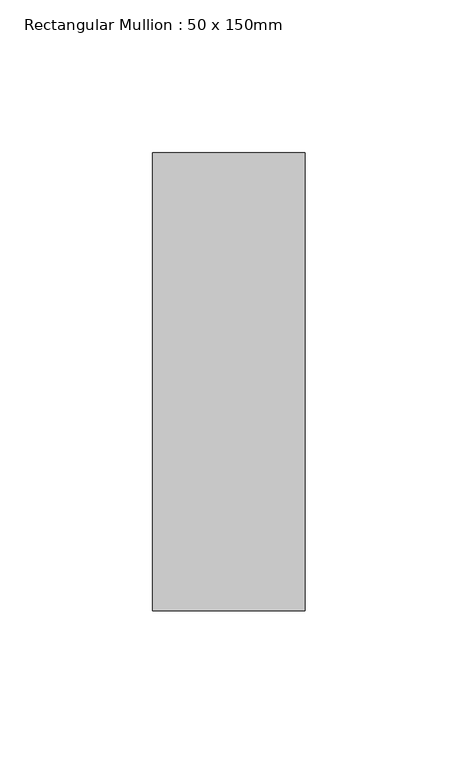
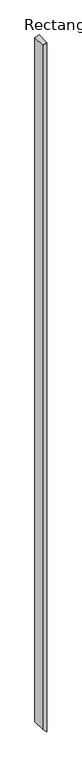
"""IFC4 building model written with IfcOpenShell, lengths in millimetres: member geometry, Rectangular Mullion : 50 x 150mm."""

from ifc_helpers import new_model, si_unit, frame, origin, place, context, project, spatial, polyline, outline, extrude, source, transform, mapped, element, save


def rectangular_mullion_50_x_150mm_f4970be0(model_context):
    return source(origin(), model_context, "Body", "SweptSolid", [
        extrude(outline(polyline([(0.0, 0.0), (-16.6341861, -50.0), (-8187.8662042, -50.0), (-8234.9396963, 0.0), (0.0, 0.0)])), frame((0.0, -75.0, 0.0), z_axis=(0.0, 1.0, 0.0), x_axis=(0.0, 0.0, 1.0)), (0.0, 0.0, 1.0), 150.0),
    ])


if __name__ == "__main__":
    model = new_model("IFC4")
    model_context = context("Model", 3, world=origin())
    ifc_project = project(units=[si_unit("LENGTHUNIT", "METRE", prefix="MILLI")], contexts=[model_context])
    site = spatial("IfcSite", under=ifc_project)
    building = spatial("IfcBuilding", under=site)
    placement = place(None, origin())
    rectangular_mullion_50_x_150mm_shape = rectangular_mullion_50_x_150mm_f4970be0(model_context)
    element("IfcMember", 1, ObjectType="Rectangular Mullion : 50 x 150mm", at=placement, inside=building, context=model_context, shape_type="MappedRepresentation", body=[
        mapped(rectangular_mullion_50_x_150mm_shape, transform((0.0, 0.0, 0.0), x_axis=(1.0, 0.0, 0.0), y_axis=(0.0, 1.0, 0.0), z_axis=(0.0, 0.0, 1.0))),
    ])
    save(model, "model.ifc")

# Revit data of these elements
# Type "Rectangular Mullion : 50 x 150mm"
#   built-in parameter 1007304 = 0.492126 (stored number, unit not read)
#   built-in parameter 1007301 = 0.082021 (stored number, unit not read)
#   built-in parameter 1007300 = 0.082021 (stored number, unit not read)
# Element 1 (IfcMember, "Rectangular Mullion : 50 x 150mm")
#   Materials on its faces: "Metal - Aluminium"
# Materials
#   "Metal - Aluminium": class "Metal", colour RGB 247 247 247, transparency 0
